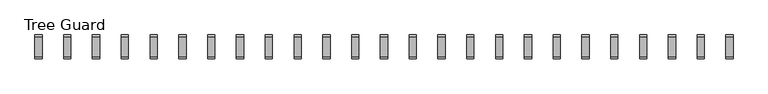
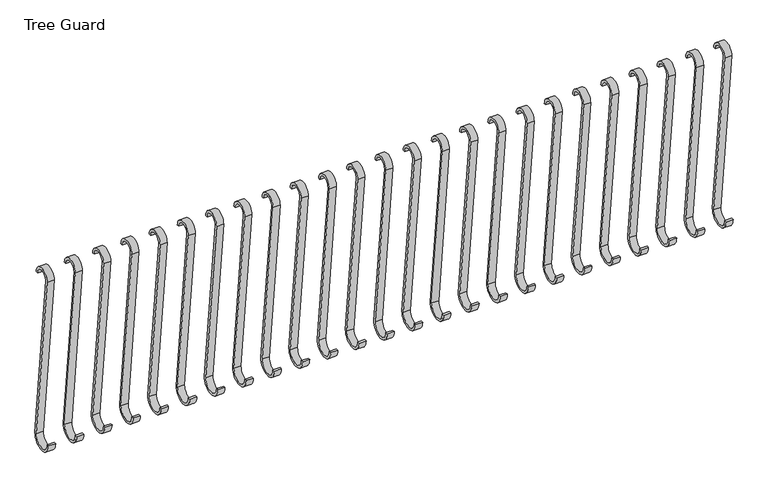
"""IFC4 building model written with IfcOpenShell, lengths in millimetres: railing geometry, Tree Guard."""

from ifc_helpers import new_model, si_unit, point, frame, frame_2d, origin, place, context, project, spatial, polyline, circle_curve, trimmed, segment, composite_curve, outline, extrude, source, transform, mapped, element, save


def tree_guard_682b009a(model_context):
    return source(origin(), model_context, "Body", "SweptSolid", [
        extrude(outline(composite_curve([segment(trimmed(circle_curve(frame_2d((-6558.5869829, 990.6)), 38.1), [point((-6520.4869829, 990.6))], [point((-6596.6815376, 991.2441257))], True, "CARTESIAN"), True, "CONTINUOUS"), segment(polyline([(-6596.6815376, 991.2441257), (-6495.0912061, 64.2323509)]), True, "CONTINUOUS"), segment(trimmed(circle_curve(frame_2d((-6558.5869829, 63.5)), 63.5), [point((-6495.0912061, 64.2323509))], [point((-6622.0869829, 63.5))], False, "CARTESIAN"), True, "CONTINUOUS"), segment(polyline([(-6622.0869829, 63.5), (-6609.3869829, 63.5)]), True, "CONTINUOUS"), segment(trimmed(circle_curve(frame_2d((-6558.5869829, 63.5)), 50.8), [point((-6609.3869829, 63.5))], [point((-6507.7869829, 63.5))], True, "CARTESIAN"), True, "CONTINUOUS"), segment(polyline([(-6507.7869829, 63.5), (-6609.3869829, 990.6)]), True, "CONTINUOUS"), segment(trimmed(circle_curve(frame_2d((-6558.5869829, 990.6)), 50.8), [point((-6609.3869829, 990.6))], [point((-6507.7869829, 990.6))], False, "CARTESIAN"), True, "CONTINUOUS"), segment(polyline([(-6507.7869829, 990.6), (-6520.4869829, 990.6)]), True, "CONTINUOUS")], self_intersect=False)), frame((2581.108432, 0.0, 0.0), z_axis=(1.0, 0.0, 0.0), x_axis=(0.0, 1.0, 0.0)), (0.0, 0.0, 1.0), 38.1),
        extrude(outline(composite_curve([segment(trimmed(circle_curve(frame_2d((-6558.5869829, 990.6)), 38.1), [point((-6520.4869829, 990.6))], [point((-6596.6815376, 991.2441257))], True, "CARTESIAN"), True, "CONTINUOUS"), segment(polyline([(-6596.6815376, 991.2441257), (-6495.0912061, 64.2323509)]), True, "CONTINUOUS"), segment(trimmed(circle_curve(frame_2d((-6558.5869829, 63.5)), 63.5), [point((-6495.0912061, 64.2323509))], [point((-6622.0869829, 63.5))], False, "CARTESIAN"), True, "CONTINUOUS"), segment(polyline([(-6622.0869829, 63.5), (-6609.3869829, 63.5)]), True, "CONTINUOUS"), segment(trimmed(circle_curve(frame_2d((-6558.5869829, 63.5)), 50.8), [point((-6609.3869829, 63.5))], [point((-6507.7869829, 63.5))], True, "CARTESIAN"), True, "CONTINUOUS"), segment(polyline([(-6507.7869829, 63.5), (-6609.3869829, 990.6)]), True, "CONTINUOUS"), segment(trimmed(circle_curve(frame_2d((-6558.5869829, 990.6)), 50.8), [point((-6609.3869829, 990.6))], [point((-6507.7869829, 990.6))], False, "CARTESIAN"), True, "CONTINUOUS"), segment(polyline([(-6507.7869829, 990.6), (-6520.4869829, 990.6)]), True, "CONTINUOUS")], self_intersect=False)), frame((2733.508432, 0.0, 0.0), z_axis=(1.0, 0.0, 0.0), x_axis=(0.0, 1.0, 0.0)), (0.0, 0.0, 1.0), 38.1),
        extrude(outline(composite_curve([segment(trimmed(circle_curve(frame_2d((-6558.5869829, 990.6)), 38.1), [point((-6520.4869829, 990.6))], [point((-6596.6815376, 991.2441257))], True, "CARTESIAN"), True, "CONTINUOUS"), segment(polyline([(-6596.6815376, 991.2441257), (-6495.0912061, 64.2323509)]), True, "CONTINUOUS"), segment(trimmed(circle_curve(frame_2d((-6558.5869829, 63.5)), 63.5), [point((-6495.0912061, 64.2323509))], [point((-6622.0869829, 63.5))], False, "CARTESIAN"), True, "CONTINUOUS"), segment(polyline([(-6622.0869829, 63.5), (-6609.3869829, 63.5)]), True, "CONTINUOUS"), segment(trimmed(circle_curve(frame_2d((-6558.5869829, 63.5)), 50.8), [point((-6609.3869829, 63.5))], [point((-6507.7869829, 63.5))], True, "CARTESIAN"), True, "CONTINUOUS"), segment(polyline([(-6507.7869829, 63.5), (-6609.3869829, 990.6)]), True, "CONTINUOUS"), segment(trimmed(circle_curve(frame_2d((-6558.5869829, 990.6)), 50.8), [point((-6609.3869829, 990.6))], [point((-6507.7869829, 990.6))], False, "CARTESIAN"), True, "CONTINUOUS"), segment(polyline([(-6507.7869829, 990.6), (-6520.4869829, 990.6)]), True, "CONTINUOUS")], self_intersect=False)), frame((2885.908432, 0.0, 0.0), z_axis=(1.0, 0.0, 0.0), x_axis=(0.0, 1.0, 0.0)), (0.0, 0.0, 1.0), 38.1),
        extrude(outline(composite_curve([segment(trimmed(circle_curve(frame_2d((-6558.5869829, 990.6)), 38.1), [point((-6520.4869829, 990.6))], [point((-6596.6815376, 991.2441257))], True, "CARTESIAN"), True, "CONTINUOUS"), segment(polyline([(-6596.6815376, 991.2441257), (-6495.0912061, 64.2323509)]), True, "CONTINUOUS"), segment(trimmed(circle_curve(frame_2d((-6558.5869829, 63.5)), 63.5), [point((-6495.0912061, 64.2323509))], [point((-6622.0869829, 63.5))], False, "CARTESIAN"), True, "CONTINUOUS"), segment(polyline([(-6622.0869829, 63.5), (-6609.3869829, 63.5)]), True, "CONTINUOUS"), segment(trimmed(circle_curve(frame_2d((-6558.5869829, 63.5)), 50.8), [point((-6609.3869829, 63.5))], [point((-6507.7869829, 63.5))], True, "CARTESIAN"), True, "CONTINUOUS"), segment(polyline([(-6507.7869829, 63.5), (-6609.3869829, 990.6)]), True, "CONTINUOUS"), segment(trimmed(circle_curve(frame_2d((-6558.5869829, 990.6)), 50.8), [point((-6609.3869829, 990.6))], [point((-6507.7869829, 990.6))], False, "CARTESIAN"), True, "CONTINUOUS"), segment(polyline([(-6507.7869829, 990.6), (-6520.4869829, 990.6)]), True, "CONTINUOUS")], self_intersect=False)), frame((3038.308432, 0.0, 0.0), z_axis=(1.0, 0.0, 0.0), x_axis=(0.0, 1.0, 0.0)), (0.0, 0.0, 1.0), 38.1),
        extrude(outline(composite_curve([segment(trimmed(circle_curve(frame_2d((-6558.5869829, 990.6)), 38.1), [point((-6520.4869829, 990.6))], [point((-6596.6815376, 991.2441257))], True, "CARTESIAN"), True, "CONTINUOUS"), segment(polyline([(-6596.6815376, 991.2441257), (-6495.0912061, 64.2323509)]), True, "CONTINUOUS"), segment(trimmed(circle_curve(frame_2d((-6558.5869829, 63.5)), 63.5), [point((-6495.0912061, 64.2323509))], [point((-6622.0869829, 63.5))], False, "CARTESIAN"), True, "CONTINUOUS"), segment(polyline([(-6622.0869829, 63.5), (-6609.3869829, 63.5)]), True, "CONTINUOUS"), segment(trimmed(circle_curve(frame_2d((-6558.5869829, 63.5)), 50.8), [point((-6609.3869829, 63.5))], [point((-6507.7869829, 63.5))], True, "CARTESIAN"), True, "CONTINUOUS"), segment(polyline([(-6507.7869829, 63.5), (-6609.3869829, 990.6)]), True, "CONTINUOUS"), segment(trimmed(circle_curve(frame_2d((-6558.5869829, 990.6)), 50.8), [point((-6609.3869829, 990.6))], [point((-6507.7869829, 990.6))], False, "CARTESIAN"), True, "CONTINUOUS"), segment(polyline([(-6507.7869829, 990.6), (-6520.4869829, 990.6)]), True, "CONTINUOUS")], self_intersect=False)), frame((3190.708432, 0.0, 0.0), z_axis=(1.0, 0.0, 0.0), x_axis=(0.0, 1.0, 0.0)), (0.0, 0.0, 1.0), 38.1),
        extrude(outline(composite_curve([segment(trimmed(circle_curve(frame_2d((-6558.5869829, 990.6)), 38.1), [point((-6520.4869829, 990.6))], [point((-6596.6815376, 991.2441257))], True, "CARTESIAN"), True, "CONTINUOUS"), segment(polyline([(-6596.6815376, 991.2441257), (-6495.0912061, 64.2323509)]), True, "CONTINUOUS"), segment(trimmed(circle_curve(frame_2d((-6558.5869829, 63.5)), 63.5), [point((-6495.0912061, 64.2323509))], [point((-6622.0869829, 63.5))], False, "CARTESIAN"), True, "CONTINUOUS"), segment(polyline([(-6622.0869829, 63.5), (-6609.3869829, 63.5)]), True, "CONTINUOUS"), segment(trimmed(circle_curve(frame_2d((-6558.5869829, 63.5)), 50.8), [point((-6609.3869829, 63.5))], [point((-6507.7869829, 63.5))], True, "CARTESIAN"), True, "CONTINUOUS"), segment(polyline([(-6507.7869829, 63.5), (-6609.3869829, 990.6)]), True, "CONTINUOUS"), segment(trimmed(circle_curve(frame_2d((-6558.5869829, 990.6)), 50.8), [point((-6609.3869829, 990.6))], [point((-6507.7869829, 990.6))], False, "CARTESIAN"), True, "CONTINUOUS"), segment(polyline([(-6507.7869829, 990.6), (-6520.4869829, 990.6)]), True, "CONTINUOUS")], self_intersect=False)), frame((3343.108432, 0.0, 0.0), z_axis=(1.0, 0.0, 0.0), x_axis=(0.0, 1.0, 0.0)), (0.0, 0.0, 1.0), 38.1),
        extrude(outline(composite_curve([segment(trimmed(circle_curve(frame_2d((-6558.5869829, 990.6)), 38.1), [point((-6520.4869829, 990.6))], [point((-6596.6815376, 991.2441257))], True, "CARTESIAN"), True, "CONTINUOUS"), segment(polyline([(-6596.6815376, 991.2441257), (-6495.0912061, 64.2323509)]), True, "CONTINUOUS"), segment(trimmed(circle_curve(frame_2d((-6558.5869829, 63.5)), 63.5), [point((-6495.0912061, 64.2323509))], [point((-6622.0869829, 63.5))], False, "CARTESIAN"), True, "CONTINUOUS"), segment(polyline([(-6622.0869829, 63.5), (-6609.3869829, 63.5)]), True, "CONTINUOUS"), segment(trimmed(circle_curve(frame_2d((-6558.5869829, 63.5)), 50.8), [point((-6609.3869829, 63.5))], [point((-6507.7869829, 63.5))], True, "CARTESIAN"), True, "CONTINUOUS"), segment(polyline([(-6507.7869829, 63.5), (-6609.3869829, 990.6)]), True, "CONTINUOUS"), segment(trimmed(circle_curve(frame_2d((-6558.5869829, 990.6)), 50.8), [point((-6609.3869829, 990.6))], [point((-6507.7869829, 990.6))], False, "CARTESIAN"), True, "CONTINUOUS"), segment(polyline([(-6507.7869829, 990.6), (-6520.4869829, 990.6)]), True, "CONTINUOUS")], self_intersect=False)), frame((3495.508432, 0.0, 0.0), z_axis=(1.0, 0.0, 0.0), x_axis=(0.0, 1.0, 0.0)), (0.0, 0.0, 1.0), 38.1),
        extrude(outline(composite_curve([segment(trimmed(circle_curve(frame_2d((-6558.5869829, 990.6)), 38.1), [point((-6520.4869829, 990.6))], [point((-6596.6815376, 991.2441257))], True, "CARTESIAN"), True, "CONTINUOUS"), segment(polyline([(-6596.6815376, 991.2441257), (-6495.0912061, 64.2323509)]), True, "CONTINUOUS"), segment(trimmed(circle_curve(frame_2d((-6558.5869829, 63.5)), 63.5), [point((-6495.0912061, 64.2323509))], [point((-6622.0869829, 63.5))], False, "CARTESIAN"), True, "CONTINUOUS"), segment(polyline([(-6622.0869829, 63.5), (-6609.3869829, 63.5)]), True, "CONTINUOUS"), segment(trimmed(circle_curve(frame_2d((-6558.5869829, 63.5)), 50.8), [point((-6609.3869829, 63.5))], [point((-6507.7869829, 63.5))], True, "CARTESIAN"), True, "CONTINUOUS"), segment(polyline([(-6507.7869829, 63.5), (-6609.3869829, 990.6)]), True, "CONTINUOUS"), segment(trimmed(circle_curve(frame_2d((-6558.5869829, 990.6)), 50.8), [point((-6609.3869829, 990.6))], [point((-6507.7869829, 990.6))], False, "CARTESIAN"), True, "CONTINUOUS"), segment(polyline([(-6507.7869829, 990.6), (-6520.4869829, 990.6)]), True, "CONTINUOUS")], self_intersect=False)), frame((3647.908432, 0.0, 0.0), z_axis=(1.0, 0.0, 0.0), x_axis=(0.0, 1.0, 0.0)), (0.0, 0.0, 1.0), 38.1),
        extrude(outline(composite_curve([segment(trimmed(circle_curve(frame_2d((-6558.5869829, 990.6)), 38.1), [point((-6520.4869829, 990.6))], [point((-6596.6815376, 991.2441257))], True, "CARTESIAN"), True, "CONTINUOUS"), segment(polyline([(-6596.6815376, 991.2441257), (-6495.0912061, 64.2323509)]), True, "CONTINUOUS"), segment(trimmed(circle_curve(frame_2d((-6558.5869829, 63.5)), 63.5), [point((-6495.0912061, 64.2323509))], [point((-6622.0869829, 63.5))], False, "CARTESIAN"), True, "CONTINUOUS"), segment(polyline([(-6622.0869829, 63.5), (-6609.3869829, 63.5)]), True, "CONTINUOUS"), segment(trimmed(circle_curve(frame_2d((-6558.5869829, 63.5)), 50.8), [point((-6609.3869829, 63.5))], [point((-6507.7869829, 63.5))], True, "CARTESIAN"), True, "CONTINUOUS"), segment(polyline([(-6507.7869829, 63.5), (-6609.3869829, 990.6)]), True, "CONTINUOUS"), segment(trimmed(circle_curve(frame_2d((-6558.5869829, 990.6)), 50.8), [point((-6609.3869829, 990.6))], [point((-6507.7869829, 990.6))], False, "CARTESIAN"), True, "CONTINUOUS"), segment(polyline([(-6507.7869829, 990.6), (-6520.4869829, 990.6)]), True, "CONTINUOUS")], self_intersect=False)), frame((3800.308432, 0.0, 0.0), z_axis=(1.0, 0.0, 0.0), x_axis=(0.0, 1.0, 0.0)), (0.0, 0.0, 1.0), 38.1),
        extrude(outline(composite_curve([segment(trimmed(circle_curve(frame_2d((-6558.5869829, 990.6)), 38.1), [point((-6520.4869829, 990.6))], [point((-6596.6815376, 991.2441257))], True, "CARTESIAN"), True, "CONTINUOUS"), segment(polyline([(-6596.6815376, 991.2441257), (-6495.0912061, 64.2323509)]), True, "CONTINUOUS"), segment(trimmed(circle_curve(frame_2d((-6558.5869829, 63.5)), 63.5), [point((-6495.0912061, 64.2323509))], [point((-6622.0869829, 63.5))], False, "CARTESIAN"), True, "CONTINUOUS"), segment(polyline([(-6622.0869829, 63.5), (-6609.3869829, 63.5)]), True, "CONTINUOUS"), segment(trimmed(circle_curve(frame_2d((-6558.5869829, 63.5)), 50.8), [point((-6609.3869829, 63.5))], [point((-6507.7869829, 63.5))], True, "CARTESIAN"), True, "CONTINUOUS"), segment(polyline([(-6507.7869829, 63.5), (-6609.3869829, 990.6)]), True, "CONTINUOUS"), segment(trimmed(circle_curve(frame_2d((-6558.5869829, 990.6)), 50.8), [point((-6609.3869829, 990.6))], [point((-6507.7869829, 990.6))], False, "CARTESIAN"), True, "CONTINUOUS"), segment(polyline([(-6507.7869829, 990.6), (-6520.4869829, 990.6)]), True, "CONTINUOUS")], self_intersect=False)), frame((3952.708432, 0.0, 0.0), z_axis=(1.0, 0.0, 0.0), x_axis=(0.0, 1.0, 0.0)), (0.0, 0.0, 1.0), 38.1),
        extrude(outline(composite_curve([segment(trimmed(circle_curve(frame_2d((-6558.5869829, 990.6)), 38.1), [point((-6520.4869829, 990.6))], [point((-6596.6815376, 991.2441257))], True, "CARTESIAN"), True, "CONTINUOUS"), segment(polyline([(-6596.6815376, 991.2441257), (-6495.0912061, 64.2323509)]), True, "CONTINUOUS"), segment(trimmed(circle_curve(frame_2d((-6558.5869829, 63.5)), 63.5), [point((-6495.0912061, 64.2323509))], [point((-6622.0869829, 63.5))], False, "CARTESIAN"), True, "CONTINUOUS"), segment(polyline([(-6622.0869829, 63.5), (-6609.3869829, 63.5)]), True, "CONTINUOUS"), segment(trimmed(circle_curve(frame_2d((-6558.5869829, 63.5)), 50.8), [point((-6609.3869829, 63.5))], [point((-6507.7869829, 63.5))], True, "CARTESIAN"), True, "CONTINUOUS"), segment(polyline([(-6507.7869829, 63.5), (-6609.3869829, 990.6)]), True, "CONTINUOUS"), segment(trimmed(circle_curve(frame_2d((-6558.5869829, 990.6)), 50.8), [point((-6609.3869829, 990.6))], [point((-6507.7869829, 990.6))], False, "CARTESIAN"), True, "CONTINUOUS"), segment(polyline([(-6507.7869829, 990.6), (-6520.4869829, 990.6)]), True, "CONTINUOUS")], self_intersect=False)), frame((4105.108432, 0.0, 0.0), z_axis=(1.0, 0.0, 0.0), x_axis=(0.0, 1.0, 0.0)), (0.0, 0.0, 1.0), 38.1),
        extrude(outline(composite_curve([segment(trimmed(circle_curve(frame_2d((-6558.5869829, 990.6)), 38.1), [point((-6520.4869829, 990.6))], [point((-6596.6815376, 991.2441257))], True, "CARTESIAN"), True, "CONTINUOUS"), segment(polyline([(-6596.6815376, 991.2441257), (-6495.0912061, 64.2323509)]), True, "CONTINUOUS"), segment(trimmed(circle_curve(frame_2d((-6558.5869829, 63.5)), 63.5), [point((-6495.0912061, 64.2323509))], [point((-6622.0869829, 63.5))], False, "CARTESIAN"), True, "CONTINUOUS"), segment(polyline([(-6622.0869829, 63.5), (-6609.3869829, 63.5)]), True, "CONTINUOUS"), segment(trimmed(circle_curve(frame_2d((-6558.5869829, 63.5)), 50.8), [point((-6609.3869829, 63.5))], [point((-6507.7869829, 63.5))], True, "CARTESIAN"), True, "CONTINUOUS"), segment(polyline([(-6507.7869829, 63.5), (-6609.3869829, 990.6)]), True, "CONTINUOUS"), segment(trimmed(circle_curve(frame_2d((-6558.5869829, 990.6)), 50.8), [point((-6609.3869829, 990.6))], [point((-6507.7869829, 990.6))], False, "CARTESIAN"), True, "CONTINUOUS"), segment(polyline([(-6507.7869829, 990.6), (-6520.4869829, 990.6)]), True, "CONTINUOUS")], self_intersect=False)), frame((4257.508432, 0.0, 0.0), z_axis=(1.0, 0.0, 0.0), x_axis=(0.0, 1.0, 0.0)), (0.0, 0.0, 1.0), 38.1),
        extrude(outline(composite_curve([segment(trimmed(circle_curve(frame_2d((-6558.5869829, 990.6)), 38.1), [point((-6520.4869829, 990.6))], [point((-6596.6815376, 991.2441257))], True, "CARTESIAN"), True, "CONTINUOUS"), segment(polyline([(-6596.6815376, 991.2441257), (-6495.0912061, 64.2323509)]), True, "CONTINUOUS"), segment(trimmed(circle_curve(frame_2d((-6558.5869829, 63.5)), 63.5), [point((-6495.0912061, 64.2323509))], [point((-6622.0869829, 63.5))], False, "CARTESIAN"), True, "CONTINUOUS"), segment(polyline([(-6622.0869829, 63.5), (-6609.3869829, 63.5)]), True, "CONTINUOUS"), segment(trimmed(circle_curve(frame_2d((-6558.5869829, 63.5)), 50.8), [point((-6609.3869829, 63.5))], [point((-6507.7869829, 63.5))], True, "CARTESIAN"), True, "CONTINUOUS"), segment(polyline([(-6507.7869829, 63.5), (-6609.3869829, 990.6)]), True, "CONTINUOUS"), segment(trimmed(circle_curve(frame_2d((-6558.5869829, 990.6)), 50.8), [point((-6609.3869829, 990.6))], [point((-6507.7869829, 990.6))], False, "CARTESIAN"), True, "CONTINUOUS"), segment(polyline([(-6507.7869829, 990.6), (-6520.4869829, 990.6)]), True, "CONTINUOUS")], self_intersect=False)), frame((4409.908432, 0.0, 0.0), z_axis=(1.0, 0.0, 0.0), x_axis=(0.0, 1.0, 0.0)), (0.0, 0.0, 1.0), 38.1),
        extrude(outline(composite_curve([segment(trimmed(circle_curve(frame_2d((-6558.5869829, 990.6)), 38.1), [point((-6520.4869829, 990.6))], [point((-6596.6815376, 991.2441257))], True, "CARTESIAN"), True, "CONTINUOUS"), segment(polyline([(-6596.6815376, 991.2441257), (-6495.0912061, 64.2323509)]), True, "CONTINUOUS"), segment(trimmed(circle_curve(frame_2d((-6558.5869829, 63.5)), 63.5), [point((-6495.0912061, 64.2323509))], [point((-6622.0869829, 63.5))], False, "CARTESIAN"), True, "CONTINUOUS"), segment(polyline([(-6622.0869829, 63.5), (-6609.3869829, 63.5)]), True, "CONTINUOUS"), segment(trimmed(circle_curve(frame_2d((-6558.5869829, 63.5)), 50.8), [point((-6609.3869829, 63.5))], [point((-6507.7869829, 63.5))], True, "CARTESIAN"), True, "CONTINUOUS"), segment(polyline([(-6507.7869829, 63.5), (-6609.3869829, 990.6)]), True, "CONTINUOUS"), segment(trimmed(circle_curve(frame_2d((-6558.5869829, 990.6)), 50.8), [point((-6609.3869829, 990.6))], [point((-6507.7869829, 990.6))], False, "CARTESIAN"), True, "CONTINUOUS"), segment(polyline([(-6507.7869829, 990.6), (-6520.4869829, 990.6)]), True, "CONTINUOUS")], self_intersect=False)), frame((4562.308432, 0.0, 0.0), z_axis=(1.0, 0.0, 0.0), x_axis=(0.0, 1.0, 0.0)), (0.0, 0.0, 1.0), 38.1),
        extrude(outline(composite_curve([segment(trimmed(circle_curve(frame_2d((-6558.5869829, 990.6)), 38.1), [point((-6520.4869829, 990.6))], [point((-6596.6815376, 991.2441257))], True, "CARTESIAN"), True, "CONTINUOUS"), segment(polyline([(-6596.6815376, 991.2441257), (-6495.0912061, 64.2323509)]), True, "CONTINUOUS"), segment(trimmed(circle_curve(frame_2d((-6558.5869829, 63.5)), 63.5), [point((-6495.0912061, 64.2323509))], [point((-6622.0869829, 63.5))], False, "CARTESIAN"), True, "CONTINUOUS"), segment(polyline([(-6622.0869829, 63.5), (-6609.3869829, 63.5)]), True, "CONTINUOUS"), segment(trimmed(circle_curve(frame_2d((-6558.5869829, 63.5)), 50.8), [point((-6609.3869829, 63.5))], [point((-6507.7869829, 63.5))], True, "CARTESIAN"), True, "CONTINUOUS"), segment(polyline([(-6507.7869829, 63.5), (-6609.3869829, 990.6)]), True, "CONTINUOUS"), segment(trimmed(circle_curve(frame_2d((-6558.5869829, 990.6)), 50.8), [point((-6609.3869829, 990.6))], [point((-6507.7869829, 990.6))], False, "CARTESIAN"), True, "CONTINUOUS"), segment(polyline([(-6507.7869829, 990.6), (-6520.4869829, 990.6)]), True, "CONTINUOUS")], self_intersect=False)), frame((4714.708432, 0.0, 0.0), z_axis=(1.0, 0.0, 0.0), x_axis=(0.0, 1.0, 0.0)), (0.0, 0.0, 1.0), 38.1),
        extrude(outline(composite_curve([segment(trimmed(circle_curve(frame_2d((-6558.5869829, 990.6)), 38.1), [point((-6520.4869829, 990.6))], [point((-6596.6815376, 991.2441257))], True, "CARTESIAN"), True, "CONTINUOUS"), segment(polyline([(-6596.6815376, 991.2441257), (-6495.0912061, 64.2323509)]), True, "CONTINUOUS"), segment(trimmed(circle_curve(frame_2d((-6558.5869829, 63.5)), 63.5), [point((-6495.0912061, 64.2323509))], [point((-6622.0869829, 63.5))], False, "CARTESIAN"), True, "CONTINUOUS"), segment(polyline([(-6622.0869829, 63.5), (-6609.3869829, 63.5)]), True, "CONTINUOUS"), segment(trimmed(circle_curve(frame_2d((-6558.5869829, 63.5)), 50.8), [point((-6609.3869829, 63.5))], [point((-6507.7869829, 63.5))], True, "CARTESIAN"), True, "CONTINUOUS"), segment(polyline([(-6507.7869829, 63.5), (-6609.3869829, 990.6)]), True, "CONTINUOUS"), segment(trimmed(circle_curve(frame_2d((-6558.5869829, 990.6)), 50.8), [point((-6609.3869829, 990.6))], [point((-6507.7869829, 990.6))], False, "CARTESIAN"), True, "CONTINUOUS"), segment(polyline([(-6507.7869829, 990.6), (-6520.4869829, 990.6)]), True, "CONTINUOUS")], self_intersect=False)), frame((4867.108432, 0.0, 0.0), z_axis=(1.0, 0.0, 0.0), x_axis=(0.0, 1.0, 0.0)), (0.0, 0.0, 1.0), 38.1),
        extrude(outline(composite_curve([segment(trimmed(circle_curve(frame_2d((-6558.5869829, 990.6)), 38.1), [point((-6520.4869829, 990.6))], [point((-6596.6815376, 991.2441257))], True, "CARTESIAN"), True, "CONTINUOUS"), segment(polyline([(-6596.6815376, 991.2441257), (-6495.0912061, 64.2323509)]), True, "CONTINUOUS"), segment(trimmed(circle_curve(frame_2d((-6558.5869829, 63.5)), 63.5), [point((-6495.0912061, 64.2323509))], [point((-6622.0869829, 63.5))], False, "CARTESIAN"), True, "CONTINUOUS"), segment(polyline([(-6622.0869829, 63.5), (-6609.3869829, 63.5)]), True, "CONTINUOUS"), segment(trimmed(circle_curve(frame_2d((-6558.5869829, 63.5)), 50.8), [point((-6609.3869829, 63.5))], [point((-6507.7869829, 63.5))], True, "CARTESIAN"), True, "CONTINUOUS"), segment(polyline([(-6507.7869829, 63.5), (-6609.3869829, 990.6)]), True, "CONTINUOUS"), segment(trimmed(circle_curve(frame_2d((-6558.5869829, 990.6)), 50.8), [point((-6609.3869829, 990.6))], [point((-6507.7869829, 990.6))], False, "CARTESIAN"), True, "CONTINUOUS"), segment(polyline([(-6507.7869829, 990.6), (-6520.4869829, 990.6)]), True, "CONTINUOUS")], self_intersect=False)), frame((5019.508432, 0.0, 0.0), z_axis=(1.0, 0.0, 0.0), x_axis=(0.0, 1.0, 0.0)), (0.0, 0.0, 1.0), 38.1),
        extrude(outline(composite_curve([segment(trimmed(circle_curve(frame_2d((-6558.5869829, 990.6)), 38.1), [point((-6520.4869829, 990.6))], [point((-6596.6815376, 991.2441257))], True, "CARTESIAN"), True, "CONTINUOUS"), segment(polyline([(-6596.6815376, 991.2441257), (-6495.0912061, 64.2323509)]), True, "CONTINUOUS"), segment(trimmed(circle_curve(frame_2d((-6558.5869829, 63.5)), 63.5), [point((-6495.0912061, 64.2323509))], [point((-6622.0869829, 63.5))], False, "CARTESIAN"), True, "CONTINUOUS"), segment(polyline([(-6622.0869829, 63.5), (-6609.3869829, 63.5)]), True, "CONTINUOUS"), segment(trimmed(circle_curve(frame_2d((-6558.5869829, 63.5)), 50.8), [point((-6609.3869829, 63.5))], [point((-6507.7869829, 63.5))], True, "CARTESIAN"), True, "CONTINUOUS"), segment(polyline([(-6507.7869829, 63.5), (-6609.3869829, 990.6)]), True, "CONTINUOUS"), segment(trimmed(circle_curve(frame_2d((-6558.5869829, 990.6)), 50.8), [point((-6609.3869829, 990.6))], [point((-6507.7869829, 990.6))], False, "CARTESIAN"), True, "CONTINUOUS"), segment(polyline([(-6507.7869829, 990.6), (-6520.4869829, 990.6)]), True, "CONTINUOUS")], self_intersect=False)), frame((5171.908432, 0.0, 0.0), z_axis=(1.0, 0.0, 0.0), x_axis=(0.0, 1.0, 0.0)), (0.0, 0.0, 1.0), 38.1),
        extrude(outline(composite_curve([segment(trimmed(circle_curve(frame_2d((-6558.5869829, 990.6)), 38.1), [point((-6520.4869829, 990.6))], [point((-6596.6815376, 991.2441257))], True, "CARTESIAN"), True, "CONTINUOUS"), segment(polyline([(-6596.6815376, 991.2441257), (-6495.0912061, 64.2323509)]), True, "CONTINUOUS"), segment(trimmed(circle_curve(frame_2d((-6558.5869829, 63.5)), 63.5), [point((-6495.0912061, 64.2323509))], [point((-6622.0869829, 63.5))], False, "CARTESIAN"), True, "CONTINUOUS"), segment(polyline([(-6622.0869829, 63.5), (-6609.3869829, 63.5)]), True, "CONTINUOUS"), segment(trimmed(circle_curve(frame_2d((-6558.5869829, 63.5)), 50.8), [point((-6609.3869829, 63.5))], [point((-6507.7869829, 63.5))], True, "CARTESIAN"), True, "CONTINUOUS"), segment(polyline([(-6507.7869829, 63.5), (-6609.3869829, 990.6)]), True, "CONTINUOUS"), segment(trimmed(circle_curve(frame_2d((-6558.5869829, 990.6)), 50.8), [point((-6609.3869829, 990.6))], [point((-6507.7869829, 990.6))], False, "CARTESIAN"), True, "CONTINUOUS"), segment(polyline([(-6507.7869829, 990.6), (-6520.4869829, 990.6)]), True, "CONTINUOUS")], self_intersect=False)), frame((5324.308432, 0.0, 0.0), z_axis=(1.0, 0.0, 0.0), x_axis=(0.0, 1.0, 0.0)), (0.0, 0.0, 1.0), 38.1),
        extrude(outline(composite_curve([segment(trimmed(circle_curve(frame_2d((-6558.5869829, 990.6)), 38.1), [point((-6520.4869829, 990.6))], [point((-6596.6815376, 991.2441257))], True, "CARTESIAN"), True, "CONTINUOUS"), segment(polyline([(-6596.6815376, 991.2441257), (-6495.0912061, 64.2323509)]), True, "CONTINUOUS"), segment(trimmed(circle_curve(frame_2d((-6558.5869829, 63.5)), 63.5), [point((-6495.0912061, 64.2323509))], [point((-6622.0869829, 63.5))], False, "CARTESIAN"), True, "CONTINUOUS"), segment(polyline([(-6622.0869829, 63.5), (-6609.3869829, 63.5)]), True, "CONTINUOUS"), segment(trimmed(circle_curve(frame_2d((-6558.5869829, 63.5)), 50.8), [point((-6609.3869829, 63.5))], [point((-6507.7869829, 63.5))], True, "CARTESIAN"), True, "CONTINUOUS"), segment(polyline([(-6507.7869829, 63.5), (-6609.3869829, 990.6)]), True, "CONTINUOUS"), segment(trimmed(circle_curve(frame_2d((-6558.5869829, 990.6)), 50.8), [point((-6609.3869829, 990.6))], [point((-6507.7869829, 990.6))], False, "CARTESIAN"), True, "CONTINUOUS"), segment(polyline([(-6507.7869829, 990.6), (-6520.4869829, 990.6)]), True, "CONTINUOUS")], self_intersect=False)), frame((5476.708432, 0.0, 0.0), z_axis=(1.0, 0.0, 0.0), x_axis=(0.0, 1.0, 0.0)), (0.0, 0.0, 1.0), 38.1),
        extrude(outline(composite_curve([segment(trimmed(circle_curve(frame_2d((-6558.5869829, 990.6)), 38.1), [point((-6520.4869829, 990.6))], [point((-6596.6815376, 991.2441257))], True, "CARTESIAN"), True, "CONTINUOUS"), segment(polyline([(-6596.6815376, 991.2441257), (-6495.0912061, 64.2323509)]), True, "CONTINUOUS"), segment(trimmed(circle_curve(frame_2d((-6558.5869829, 63.5)), 63.5), [point((-6495.0912061, 64.2323509))], [point((-6622.0869829, 63.5))], False, "CARTESIAN"), True, "CONTINUOUS"), segment(polyline([(-6622.0869829, 63.5), (-6609.3869829, 63.5)]), True, "CONTINUOUS"), segment(trimmed(circle_curve(frame_2d((-6558.5869829, 63.5)), 50.8), [point((-6609.3869829, 63.5))], [point((-6507.7869829, 63.5))], True, "CARTESIAN"), True, "CONTINUOUS"), segment(polyline([(-6507.7869829, 63.5), (-6609.3869829, 990.6)]), True, "CONTINUOUS"), segment(trimmed(circle_curve(frame_2d((-6558.5869829, 990.6)), 50.8), [point((-6609.3869829, 990.6))], [point((-6507.7869829, 990.6))], False, "CARTESIAN"), True, "CONTINUOUS"), segment(polyline([(-6507.7869829, 990.6), (-6520.4869829, 990.6)]), True, "CONTINUOUS")], self_intersect=False)), frame((5629.108432, 0.0, 0.0), z_axis=(1.0, 0.0, 0.0), x_axis=(0.0, 1.0, 0.0)), (0.0, 0.0, 1.0), 38.1),
        extrude(outline(composite_curve([segment(trimmed(circle_curve(frame_2d((-6558.5869829, 990.6)), 38.1), [point((-6520.4869829, 990.6))], [point((-6596.6815376, 991.2441257))], True, "CARTESIAN"), True, "CONTINUOUS"), segment(polyline([(-6596.6815376, 991.2441257), (-6495.0912061, 64.2323509)]), True, "CONTINUOUS"), segment(trimmed(circle_curve(frame_2d((-6558.5869829, 63.5)), 63.5), [point((-6495.0912061, 64.2323509))], [point((-6622.0869829, 63.5))], False, "CARTESIAN"), True, "CONTINUOUS"), segment(polyline([(-6622.0869829, 63.5), (-6609.3869829, 63.5)]), True, "CONTINUOUS"), segment(trimmed(circle_curve(frame_2d((-6558.5869829, 63.5)), 50.8), [point((-6609.3869829, 63.5))], [point((-6507.7869829, 63.5))], True, "CARTESIAN"), True, "CONTINUOUS"), segment(polyline([(-6507.7869829, 63.5), (-6609.3869829, 990.6)]), True, "CONTINUOUS"), segment(trimmed(circle_curve(frame_2d((-6558.5869829, 990.6)), 50.8), [point((-6609.3869829, 990.6))], [point((-6507.7869829, 990.6))], False, "CARTESIAN"), True, "CONTINUOUS"), segment(polyline([(-6507.7869829, 990.6), (-6520.4869829, 990.6)]), True, "CONTINUOUS")], self_intersect=False)), frame((5781.508432, 0.0, 0.0), z_axis=(1.0, 0.0, 0.0), x_axis=(0.0, 1.0, 0.0)), (0.0, 0.0, 1.0), 38.1),
        extrude(outline(composite_curve([segment(trimmed(circle_curve(frame_2d((-6558.5869829, 990.6)), 38.1), [point((-6520.4869829, 990.6))], [point((-6596.6815376, 991.2441257))], True, "CARTESIAN"), True, "CONTINUOUS"), segment(polyline([(-6596.6815376, 991.2441257), (-6495.0912061, 64.2323509)]), True, "CONTINUOUS"), segment(trimmed(circle_curve(frame_2d((-6558.5869829, 63.5)), 63.5), [point((-6495.0912061, 64.2323509))], [point((-6622.0869829, 63.5))], False, "CARTESIAN"), True, "CONTINUOUS"), segment(polyline([(-6622.0869829, 63.5), (-6609.3869829, 63.5)]), True, "CONTINUOUS"), segment(trimmed(circle_curve(frame_2d((-6558.5869829, 63.5)), 50.8), [point((-6609.3869829, 63.5))], [point((-6507.7869829, 63.5))], True, "CARTESIAN"), True, "CONTINUOUS"), segment(polyline([(-6507.7869829, 63.5), (-6609.3869829, 990.6)]), True, "CONTINUOUS"), segment(trimmed(circle_curve(frame_2d((-6558.5869829, 990.6)), 50.8), [point((-6609.3869829, 990.6))], [point((-6507.7869829, 990.6))], False, "CARTESIAN"), True, "CONTINUOUS"), segment(polyline([(-6507.7869829, 990.6), (-6520.4869829, 990.6)]), True, "CONTINUOUS")], self_intersect=False)), frame((5933.908432, 0.0, 0.0), z_axis=(1.0, 0.0, 0.0), x_axis=(0.0, 1.0, 0.0)), (0.0, 0.0, 1.0), 38.1),
        extrude(outline(composite_curve([segment(trimmed(circle_curve(frame_2d((-6558.5869829, 990.6)), 38.1), [point((-6520.4869829, 990.6))], [point((-6596.6815376, 991.2441257))], True, "CARTESIAN"), True, "CONTINUOUS"), segment(polyline([(-6596.6815376, 991.2441257), (-6495.0912061, 64.2323509)]), True, "CONTINUOUS"), segment(trimmed(circle_curve(frame_2d((-6558.5869829, 63.5)), 63.5), [point((-6495.0912061, 64.2323509))], [point((-6622.0869829, 63.5))], False, "CARTESIAN"), True, "CONTINUOUS"), segment(polyline([(-6622.0869829, 63.5), (-6609.3869829, 63.5)]), True, "CONTINUOUS"), segment(trimmed(circle_curve(frame_2d((-6558.5869829, 63.5)), 50.8), [point((-6609.3869829, 63.5))], [point((-6507.7869829, 63.5))], True, "CARTESIAN"), True, "CONTINUOUS"), segment(polyline([(-6507.7869829, 63.5), (-6609.3869829, 990.6)]), True, "CONTINUOUS"), segment(trimmed(circle_curve(frame_2d((-6558.5869829, 990.6)), 50.8), [point((-6609.3869829, 990.6))], [point((-6507.7869829, 990.6))], False, "CARTESIAN"), True, "CONTINUOUS"), segment(polyline([(-6507.7869829, 990.6), (-6520.4869829, 990.6)]), True, "CONTINUOUS")], self_intersect=False)), frame((6086.308432, 0.0, 0.0), z_axis=(1.0, 0.0, 0.0), x_axis=(0.0, 1.0, 0.0)), (0.0, 0.0, 1.0), 38.1),
        extrude(outline(composite_curve([segment(trimmed(circle_curve(frame_2d((-6558.5869829, 990.6)), 38.1), [point((-6520.4869829, 990.6))], [point((-6596.6815376, 991.2441257))], True, "CARTESIAN"), True, "CONTINUOUS"), segment(polyline([(-6596.6815376, 991.2441257), (-6495.0912061, 64.2323509)]), True, "CONTINUOUS"), segment(trimmed(circle_curve(frame_2d((-6558.5869829, 63.5)), 63.5), [point((-6495.0912061, 64.2323509))], [point((-6622.0869829, 63.5))], False, "CARTESIAN"), True, "CONTINUOUS"), segment(polyline([(-6622.0869829, 63.5), (-6609.3869829, 63.5)]), True, "CONTINUOUS"), segment(trimmed(circle_curve(frame_2d((-6558.5869829, 63.5)), 50.8), [point((-6609.3869829, 63.5))], [point((-6507.7869829, 63.5))], True, "CARTESIAN"), True, "CONTINUOUS"), segment(polyline([(-6507.7869829, 63.5), (-6609.3869829, 990.6)]), True, "CONTINUOUS"), segment(trimmed(circle_curve(frame_2d((-6558.5869829, 990.6)), 50.8), [point((-6609.3869829, 990.6))], [point((-6507.7869829, 990.6))], False, "CARTESIAN"), True, "CONTINUOUS"), segment(polyline([(-6507.7869829, 990.6), (-6520.4869829, 990.6)]), True, "CONTINUOUS")], self_intersect=False)), frame((6238.708432, 0.0, 0.0), z_axis=(1.0, 0.0, 0.0), x_axis=(0.0, 1.0, 0.0)), (0.0, 0.0, 1.0), 38.1),
    ])


if __name__ == "__main__":
    model = new_model("IFC4")
    model_context = context("Model", 3, world=origin())
    ifc_project = project(units=[si_unit("LENGTHUNIT", "METRE", prefix="MILLI")], contexts=[model_context])
    site = spatial("IfcSite", under=ifc_project)
    building = spatial("IfcBuilding", under=site)
    placement = place(None, origin())
    tree_guard_shape = tree_guard_682b009a(model_context)
    element("IfcRailing", 1, ObjectType="Tree Guard", at=placement, inside=building, context=model_context, shape_type="MappedRepresentation", body=[
        mapped(tree_guard_shape, transform((0.0, 0.0, 0.0), x_axis=(1.0, 0.0, 0.0), y_axis=(0.0, 1.0, 0.0), z_axis=(0.0, 0.0, 1.0))),
    ])
    save(model, "model.ifc")
